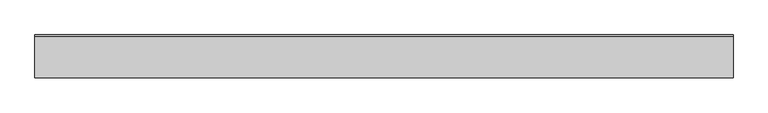
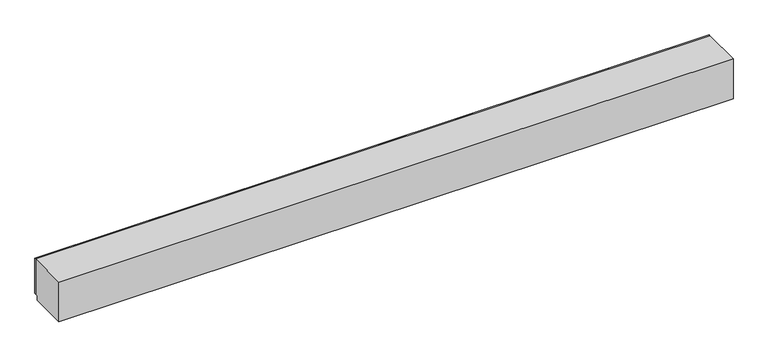
"""IFC4 building model written with IfcOpenShell, lengths in millimetres: furniture geometry, OD_CW_Base Cabinet : OD_CW_Base Cabinet."""

from ifc_helpers import new_model, si_unit, frame, origin, place, context, project, spatial, polyline, outline, extrude, source, transform, mapped, element, save


def furniture_896f4d6d(model_context):
    return source(origin(), model_context, "Body", "SweptSolid", [
        extrude(outline(polyline([(18.7377049, 228.6), (18.7377049, 254.0), (14022.9865841, 254.0), (14022.9865841, 228.6), (18.7377049, 228.6)])), frame((0.0, 0.0, 101.6), z_axis=(0.0, 0.0, 1.0), x_axis=(1.0, 0.0, 0.0)), (0.0, 0.0, 1.0), 774.7),
        extrude(outline(polyline([(228.6, 876.3), (228.6, 101.6), (177.8, 101.6), (177.8, 0.0), (-609.6, 0.0), (-609.6, 876.3), (228.6, 876.3)])), frame((18.7377049, 0.0, 0.0), z_axis=(1.0, 0.0, 0.0), x_axis=(0.0, 1.0, 0.0)), (0.0, 0.0, 1.0), 14004.2488792),
    ])


if __name__ == "__main__":
    model = new_model("IFC4")
    model_context = context("Model", 3, world=origin())
    ifc_project = project(units=[si_unit("LENGTHUNIT", "METRE", prefix="MILLI")], contexts=[model_context])
    site = spatial("IfcSite", under=ifc_project)
    building = spatial("IfcBuilding", under=site)
    placement = place(None, origin())
    furniture_shape = furniture_896f4d6d(model_context)
    element("IfcFurniture", 1, ObjectType="OD_CW_Base Cabinet : OD_CW_Base Cabinet", at=placement, inside=building, context=model_context, shape_type="MappedRepresentation", body=[
        mapped(furniture_shape, transform((0.0, 0.0, 0.0), x_axis=(1.0, 0.0, 0.0), y_axis=(0.0, 1.0, 0.0), z_axis=(0.0, 0.0, 1.0))),
    ])
    save(model, "model.ifc")

# Revit data of these elements
# Type "OD_CW_Base Cabinet : OD_CW_Base Cabinet"
#   OD_CW_Width [instance default] = 2' - 10"
#   OD_CW_Length [instance default] = 8' - 0"
#   OD_CW_Height [instance default] = 2' - 3"
#   Depth = 2' - 0"
#   Height = 3' - 0"
#   Width = 4' - 0"
#   OD_CW_Material_Front Panel [instance default] = none
#   OD_CW_Material_Body [instance default] = none
# Element 1 (IfcFurniture, "OD_CW_Base Cabinet : OD_CW_Base Cabinet")
#   OD_CW_Length = 45' - 11.34838"
#   OD_CW_Height = 2' - 10 1/2"
#   OD_CW_Material_Front Panel = WOOD-OAKFIRE
#   OD_CW_Material_Body = WOOD-OAKFIRE
#   Materials on its faces: "WOOD-OAKFIRE"
# Materials
#   "WOOD-OAKFIRE": class "Wood", colour RGB 198 202 183, transparency 0, Description = "Generic wood", Cost = 0
